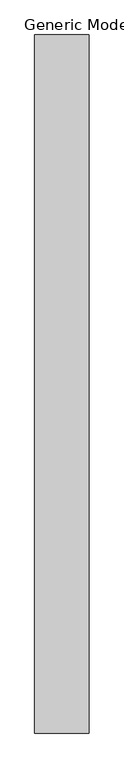
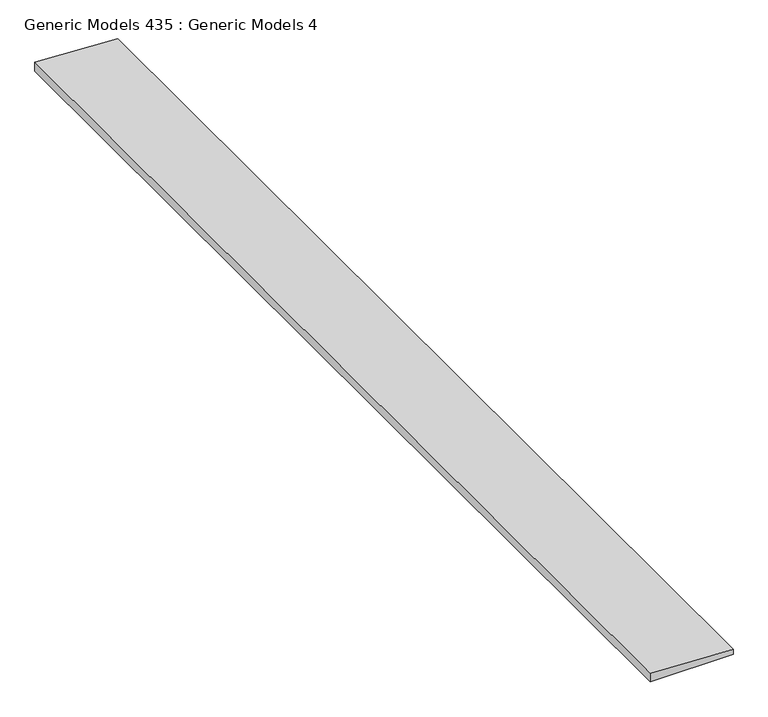
"""IFC4 building model written with IfcOpenShell, lengths in millimetres: proxy geometry, Generic Models 435 : Generic Models 4."""

import ifcopenshell
import ifcopenshell.guid

model = None  # the IFC model being written
_history = None  # IfcOwnerHistory: only IFC2X3 demands one
_inside = {}  # id of a spatial element -> (the spatial element, [elements in it])
_under = {}  # id of a project, library or spatial element -> (it, [spatial elements below it])
_declared = {}  # id of a project -> (the project, [libraries it declares])
_typed = {}  # id of a type object -> (the type object, [elements of that type])
_made_of = {}  # id of a material, layer set ... -> (it, [elements and type objects made of it])


def new_model(schema):
    """Start an empty IFC model of exactly this schema.

    Asked for "IFC4X3", IfcOpenShell would pick the latest addendum, in which some entities
    have other attributes; the version numbers below select the first issue.
    IFC2X3 requires an IfcOwnerHistory on every rooted entity: one is made here for all.
    """
    global model, _history
    if schema == "IFC4X3":
        model = ifcopenshell.file(schema_version=(4, 3, 0, 0))
    else:
        model = ifcopenshell.file(schema=schema)
    _inside.clear()
    _under.clear()
    _declared.clear()
    _typed.clear()
    _made_of.clear()
    _history = None
    if model.schema == "IFC2X3":
        org = make("IfcOrganization", Name="unknown")
        user = make(
            "IfcPersonAndOrganization",
            ThePerson=make("IfcPerson", FamilyName="unknown"),
            TheOrganization=org,
        )
        app = make(
            "IfcApplication",
            ApplicationDeveloper=org,
            Version="unknown",
            ApplicationFullName="unknown",
            ApplicationIdentifier="unknown",
        )
        _history = make(
            "IfcOwnerHistory",
            OwningUser=user,
            OwningApplication=app,
            ChangeAction="ADDED",
            CreationDate=0,
        )
    return model


def make(cls, **values):
    """One entity of the class cls with the attributes given. An attribute that is None is left unset."""
    return model.create_entity(
        cls, **{name: value for name, value in values.items() if value is not None}
    )


def rooted(cls, **values):
    """An entity with a GlobalId (a new one), such as an element, a storey or a relation."""
    return make(cls, GlobalId=ifcopenshell.guid.new(), OwnerHistory=_history, **values)


def si_unit(unit_type, name, prefix=None):
    """IfcSIUnit, for example si_unit("LENGTHUNIT", "METRE", prefix="MILLI")."""
    return make("IfcSIUnit", UnitType=unit_type, Prefix=prefix, Name=name)


def assignment(units):
    """IfcUnitAssignment: the units of a project."""
    return None if units is None else make("IfcUnitAssignment", Units=units)


def point(xyz):
    """IfcCartesianPoint."""
    return None if xyz is None else make("IfcCartesianPoint", Coordinates=xyz)


def direction(xyz):
    """IfcDirection."""
    return None if xyz is None else make("IfcDirection", DirectionRatios=xyz)


def frame(location, z_axis=None, x_axis=None):
    """IfcAxis2Placement3D, a coordinate frame: its origin and axes. An axis left out is left unset."""
    return make(
        "IfcAxis2Placement3D",
        Location=point(location),
        Axis=direction(z_axis),
        RefDirection=direction(x_axis),
    )


def origin():
    """The frame at (0, 0, 0) with its axes left unset."""
    return frame((0.0, 0.0, 0.0))


def place(relative_to, where):
    """IfcLocalPlacement: puts the frame where relative to a parent placement (None: the world)."""
    return make(
        "IfcLocalPlacement", PlacementRelTo=relative_to, RelativePlacement=where
    )


def context(
    kind, dimensions, precision=None, world=None, true_north=None, identifier=None
):
    """IfcGeometricRepresentationContext, for example the 3D "Model" context."""
    return make(
        "IfcGeometricRepresentationContext",
        ContextIdentifier=identifier,
        ContextType=kind,
        CoordinateSpaceDimension=dimensions,
        Precision=precision,
        WorldCoordinateSystem=world,
        TrueNorth=true_north,
    )


def project(units=None, contexts=None):
    """IfcProject with its units and contexts."""
    return rooted(
        "IfcProject",
        Name="project",
        RepresentationContexts=contexts,
        UnitsInContext=assignment(units),
    )


def spatial(cls, under=None, at=None, **own):
    """A site, building, storey or space (cls), placed at a placement, below another one or the project."""
    s = rooted(cls, ObjectPlacement=at, **own)
    if under is not None:
        _under.setdefault(under.id(), (under, []))[1].append(s)
    return s


def polyline(points):
    """IfcPolyline through the points."""
    return make("IfcPolyline", Points=[point(p) for p in points])


def outline(outer, holes=None, kind="AREA"):
    """IfcArbitraryClosedProfileDef: a profile drawn as a closed curve; with holes, ...WithVoids."""
    if holes is None:
        return make("IfcArbitraryClosedProfileDef", ProfileType=kind, OuterCurve=outer)
    return make(
        "IfcArbitraryProfileDefWithVoids",
        ProfileType=kind,
        OuterCurve=outer,
        InnerCurves=holes,
    )


def extrude(swept, where, along, depth):
    """IfcExtrudedAreaSolid: the profile swept, set in the frame where, extruded along a direction by depth."""
    return make(
        "IfcExtrudedAreaSolid",
        SweptArea=swept,
        Position=where,
        ExtrudedDirection=direction(along),
        Depth=depth,
    )


def shape(context_of_items, identifier, shape_type, items):
    """IfcShapeRepresentation: the items that make up one representation, for example the "Body"."""
    return make(
        "IfcShapeRepresentation",
        ContextOfItems=context_of_items,
        RepresentationIdentifier=identifier,
        RepresentationType=shape_type,
        Items=items,
    )


def source(mapping_origin, context_of_items, identifier, shape_type, items):
    """IfcRepresentationMap: a shape defined once, which mapped items show again and again."""
    return make(
        "IfcRepresentationMap",
        MappingOrigin=mapping_origin,
        MappedRepresentation=shape(context_of_items, identifier, shape_type, items),
    )


def transform(
    local_origin,
    x_axis=None,
    y_axis=None,
    z_axis=None,
    scale=None,
    scale2=None,
    scale3=None,
    uniform=True,
):
    """IfcCartesianTransformationOperator3D, or its non-uniform kind. x_axis, y_axis, z_axis: its Axis1, 2, 3."""
    if uniform:
        return make(
            "IfcCartesianTransformationOperator3D",
            Axis1=direction(x_axis),
            Axis2=direction(y_axis),
            LocalOrigin=point(local_origin),
            Scale=scale,
            Axis3=direction(z_axis),
        )
    return make(
        "IfcCartesianTransformationOperator3DnonUniform",
        Axis1=direction(x_axis),
        Axis2=direction(y_axis),
        LocalOrigin=point(local_origin),
        Scale=scale,
        Axis3=direction(z_axis),
        Scale2=scale2,
        Scale3=scale3,
    )


def mapped(mapping_source, mapping_target):
    """IfcMappedItem: shows the shape of a source again, moved by a transform."""
    return make(
        "IfcMappedItem", MappingSource=mapping_source, MappingTarget=mapping_target
    )


def made_of(thing, what):
    """Note that an element or type object is made of a material, layer set ...; save() writes the relation."""
    if what is not None:
        _made_of.setdefault(what.id(), (what, []))[1].append(thing)
    return thing


def element(
    cls,
    number,
    at=None,
    inside=None,
    cuts=None,
    type_object=None,
    material=None,
    context=None,
    identifier="Body",
    shape_type=None,
    held_by="IfcProductDefinitionShape",
    body=None,
    shapes=None,
    **own,
):
    """One element of the class cls, such as IfcWall. Its Tag is "e" and its number.

    at: its placement. inside: the storey or other place that contains it. cuts: it is an
    opening in that element (IfcRelVoidsElement). A single representation is given by context,
    identifier, shape_type and body (its items); several are given by shapes. held_by: the class
    of the entity that holds the representations. save() writes the other relations.
    """
    e = rooted(cls, Tag="e%d" % number, ObjectPlacement=at, **own)
    if body is not None:
        shapes = [shape(context, identifier, shape_type, body)]
    if shapes is not None:
        e.Representation = make(held_by, Representations=shapes)
    if inside is not None:
        _inside.setdefault(inside.id(), (inside, []))[1].append(e)
    if cuts is not None:
        rooted(
            "IfcRelVoidsElement", RelatingBuildingElement=cuts, RelatedOpeningElement=e
        )
    if type_object is not None:
        _typed.setdefault(type_object.id(), (type_object, []))[1].append(e)
    return made_of(e, material)


def aggregate(whole, parts):
    """IfcRelAggregates: a whole, such as a stair, and the parts it consists of."""
    return rooted("IfcRelAggregates", RelatingObject=whole, RelatedObjects=parts)


def save(model, path):
    """Write the relations noted so far, then the file.

    IfcRelAggregates (storeys below a building ...), IfcRelContainedInSpatialStructure (elements
    in a storey), IfcRelDefinesByType, IfcRelAssociatesMaterial and IfcRelDeclares: one each for
    every whole, place, type object, material and project.
    """
    for whole, parts in _under.values():
        aggregate(whole, parts)
    for where, things in _inside.values():
        rooted(
            "IfcRelContainedInSpatialStructure",
            RelatedElements=things,
            RelatingStructure=where,
        )
    for kind, things in _typed.values():
        rooted("IfcRelDefinesByType", RelatedObjects=things, RelatingType=kind)
    for what, things in _made_of.values():
        rooted("IfcRelAssociatesMaterial", RelatedObjects=things, RelatingMaterial=what)
    for by, libraries in _declared.values():
        rooted("IfcRelDeclares", RelatingContext=by, RelatedDefinitions=libraries)
    model.write(path)


def generic_models_435_generic_models_4_aa1da846(model_context):
    return source(origin(), model_context, "Body", "SweptSolid", [
        extrude(outline(polyline([(123577.532857, 8572.3263705), (123468.2081404, 8572.3263705), (123468.2081404, 9549.3406693), (123531.523286, 9549.3406693), (123577.532857, 8572.3263705)])), frame((0.0, -5493.3230338, 0.0), z_axis=(0.0, 1.0, 0.0), x_axis=(0.0, 0.0, 1.0)), (0.0, 0.0, 1.0), 12547.6),
    ])


if __name__ == "__main__":
    model = new_model("IFC4")
    model_context = context("Model", 3, world=origin())
    ifc_project = project(units=[si_unit("LENGTHUNIT", "METRE", prefix="MILLI")], contexts=[model_context])
    site = spatial("IfcSite", under=ifc_project)
    building = spatial("IfcBuilding", under=site)
    placement = place(None, origin())
    generic_models_435_generic_models_4_shape = generic_models_435_generic_models_4_aa1da846(model_context)
    element("IfcBuildingElementProxy", 1, Name="Generic Models 435 : Generic Models 4", ObjectType="Generic Models 435 : Generic Models 4", at=placement, inside=building, context=model_context, shape_type="MappedRepresentation", body=[
        mapped(generic_models_435_generic_models_4_shape, transform((0.0, 0.0, 0.0), x_axis=(1.0, 0.0, 0.0), y_axis=(0.0, 1.0, 0.0), z_axis=(0.0, 0.0, 1.0))),
    ])
    save(model, "model.ifc")

# Revit data of these elements
# Element 1 (IfcBuildingElementProxy, "Generic Models 435 : Generic Models 4")
#   Materials on its faces: "_COMPACTED AGGREGATE BASE"
# Materials
#   "_COMPACTED AGGREGATE BASE": class "Generic", colour RGB 191 191 191, transparency 0, Cost = 0
